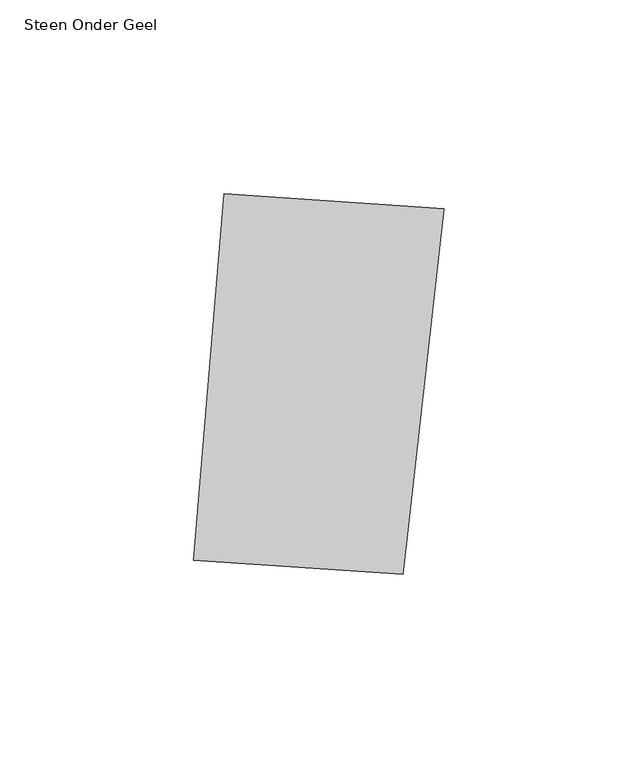
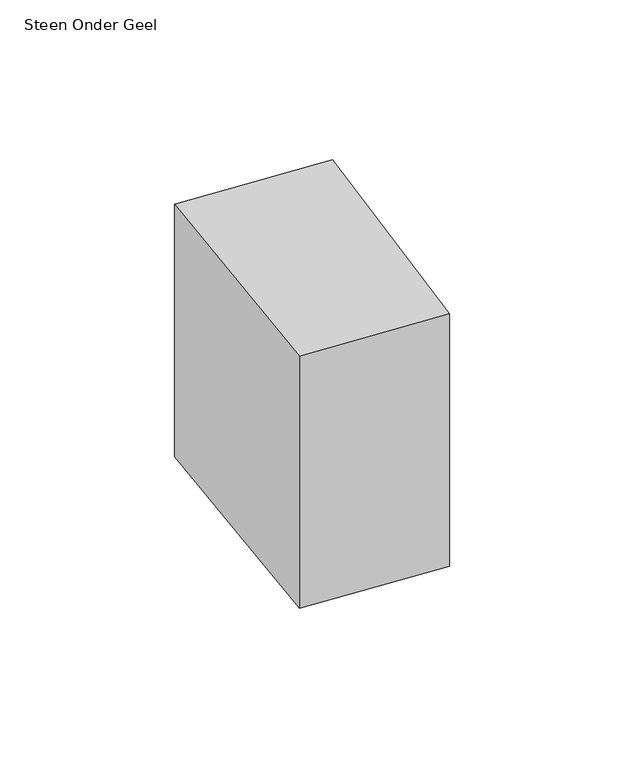
"""IFC4 building model written with IfcOpenShell, lengths in millimetres: proxy geometry, 00_GMA_steen_versie_4 : Steen Onder Geel."""

from ifc_helpers import new_model, si_unit, origin, origin_with_axes, place, context, project, spatial, polyline, outline, extrude, source, transform, mapped, element, save


def steen_onder_geel_a99939bc(model_context):
    return source(origin(), model_context, "Body", "SweptSolid", [
        extrude(outline(polyline([(105.6101224, 113.7024076), (94.9595183, 19.2049563), (40.7788766, 22.9175719), (48.6586039, 117.6012537), (105.6101224, 113.7024076)])), origin_with_axes(), (0.0, 0.0, 1.0), 100.0),
    ])


if __name__ == "__main__":
    model = new_model("IFC4")
    model_context = context("Model", 3, world=origin())
    ifc_project = project(units=[si_unit("LENGTHUNIT", "METRE", prefix="MILLI")], contexts=[model_context])
    site = spatial("IfcSite", under=ifc_project)
    building = spatial("IfcBuilding", under=site)
    placement = place(None, origin())
    steen_onder_geel_shape = steen_onder_geel_a99939bc(model_context)
    element("IfcBuildingElementProxy", 1, Name="00_GMA_steen_versie_4 : Steen Onder Geel", ObjectType="00_GMA_steen_versie_4 : Steen Onder Geel", at=placement, inside=building, context=model_context, shape_type="MappedRepresentation", body=[
        mapped(steen_onder_geel_shape, transform((0.0, 0.0, 0.0), x_axis=(1.0, 0.0, 0.0), y_axis=(0.0, 1.0, 0.0), z_axis=(0.0, 0.0, 1.0))),
    ])
    save(model, "model.ifc")

# Revit data of these elements
# Type "00_GMA_steen_versie_4 : Steen Onder Geel"
#   StootVoegHalfBoven [instance default] = 5 mm
#   StootVoegHalf [instance default] = 5 mm
#   StootVoegBreedteOnder = 10 mm
#   StootVoegBreedteBoven = 10 mm
#   Steendikte = 100 mm
#   LintVoegOnderHalf = 0 mm
#   LintVoegOnder = 0 mm
#   LintVoegBovenHalf = 5 mm
#   LintVoegBoven = 10 mm
#   materiaal = 21_steen_geel
#   MateriaalVoeg = none
#   Default Elevation = 0
# Element 1 (IfcBuildingElementProxy, "00_GMA_steen_versie_4 : Steen Onder Geel")
#   Materials on its faces: "21_steen_geel"
# Materials
#   "21_steen_geel": class "Unassigned", colour RGB 202 202 0, transparency 0, Cost = 0
